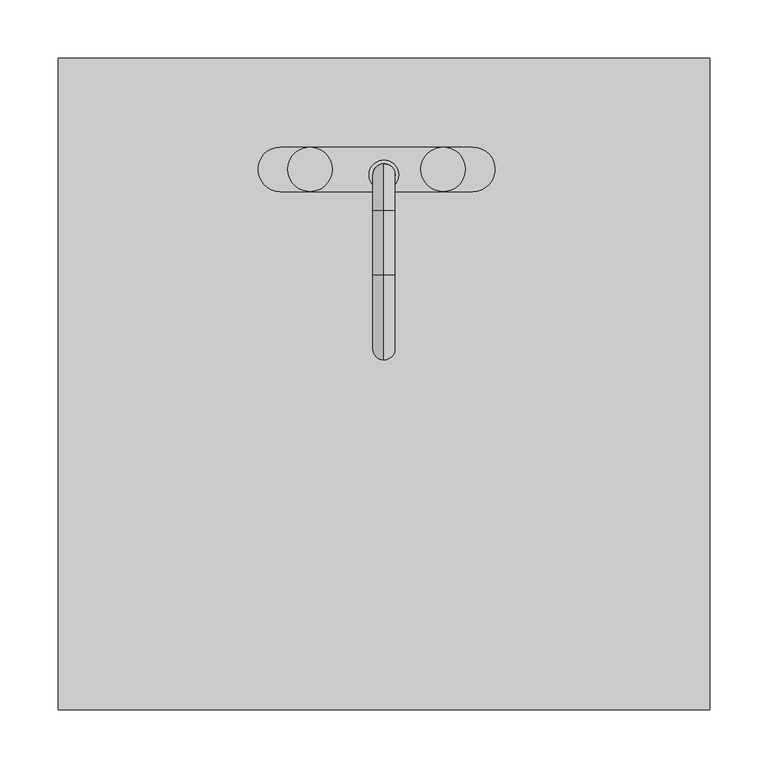
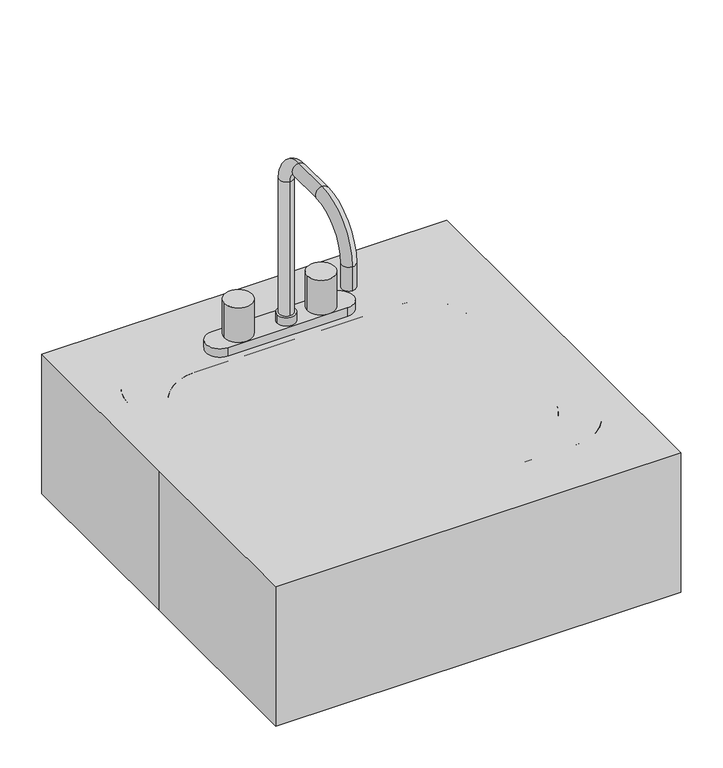
"""IFC4 building model written with IfcOpenShell, lengths in millimetres: proxy geometry, CS090 - Sink, SS, Single Compartment, 7.5x19x16 ID : CS090 - Sink, SS, Single Compartment, 7.5x19x16 ID."""

import ifcopenshell
import ifcopenshell.guid

model = None  # the IFC model being written
_history = None  # IfcOwnerHistory: only IFC2X3 demands one
_inside = {}  # id of a spatial element -> (the spatial element, [elements in it])
_under = {}  # id of a project, library or spatial element -> (it, [spatial elements below it])
_declared = {}  # id of a project -> (the project, [libraries it declares])
_typed = {}  # id of a type object -> (the type object, [elements of that type])
_made_of = {}  # id of a material, layer set ... -> (it, [elements and type objects made of it])


def new_model(schema):
    """Start an empty IFC model of exactly this schema.

    Asked for "IFC4X3", IfcOpenShell would pick the latest addendum, in which some entities
    have other attributes; the version numbers below select the first issue.
    IFC2X3 requires an IfcOwnerHistory on every rooted entity: one is made here for all.
    """
    global model, _history
    if schema == "IFC4X3":
        model = ifcopenshell.file(schema_version=(4, 3, 0, 0))
    else:
        model = ifcopenshell.file(schema=schema)
    _inside.clear()
    _under.clear()
    _declared.clear()
    _typed.clear()
    _made_of.clear()
    _history = None
    if model.schema == "IFC2X3":
        org = make("IfcOrganization", Name="unknown")
        user = make(
            "IfcPersonAndOrganization",
            ThePerson=make("IfcPerson", FamilyName="unknown"),
            TheOrganization=org,
        )
        app = make(
            "IfcApplication",
            ApplicationDeveloper=org,
            Version="unknown",
            ApplicationFullName="unknown",
            ApplicationIdentifier="unknown",
        )
        _history = make(
            "IfcOwnerHistory",
            OwningUser=user,
            OwningApplication=app,
            ChangeAction="ADDED",
            CreationDate=0,
        )
    return model


def make(cls, **values):
    """One entity of the class cls with the attributes given. An attribute that is None is left unset."""
    return model.create_entity(
        cls, **{name: value for name, value in values.items() if value is not None}
    )


def rooted(cls, **values):
    """An entity with a GlobalId (a new one), such as an element, a storey or a relation."""
    return make(cls, GlobalId=ifcopenshell.guid.new(), OwnerHistory=_history, **values)


def si_unit(unit_type, name, prefix=None):
    """IfcSIUnit, for example si_unit("LENGTHUNIT", "METRE", prefix="MILLI")."""
    return make("IfcSIUnit", UnitType=unit_type, Prefix=prefix, Name=name)


def assignment(units):
    """IfcUnitAssignment: the units of a project."""
    return None if units is None else make("IfcUnitAssignment", Units=units)


def point(xyz):
    """IfcCartesianPoint."""
    return None if xyz is None else make("IfcCartesianPoint", Coordinates=xyz)


def direction(xyz):
    """IfcDirection."""
    return None if xyz is None else make("IfcDirection", DirectionRatios=xyz)


def frame(location, z_axis=None, x_axis=None):
    """IfcAxis2Placement3D, a coordinate frame: its origin and axes. An axis left out is left unset."""
    return make(
        "IfcAxis2Placement3D",
        Location=point(location),
        Axis=direction(z_axis),
        RefDirection=direction(x_axis),
    )


def frame_2d(location, x_axis=None):
    """IfcAxis2Placement2D, a coordinate frame in the plane: its origin and x axis."""
    return make(
        "IfcAxis2Placement2D", Location=point(location), RefDirection=direction(x_axis)
    )


def origin():
    """The frame at (0, 0, 0) with its axes left unset."""
    return frame((0.0, 0.0, 0.0))


def origin_with_axes():
    """The frame at (0, 0, 0) with the z axis (0, 0, 1) and the x axis (1, 0, 0) written out."""
    return frame((0.0, 0.0, 0.0), z_axis=(0.0, 0.0, 1.0), x_axis=(1.0, 0.0, 0.0))


def origin_2d():
    """The frame at (0, 0) in the plane with its x axis left unset."""
    return frame_2d((0.0, 0.0))


def place(relative_to, where):
    """IfcLocalPlacement: puts the frame where relative to a parent placement (None: the world)."""
    return make(
        "IfcLocalPlacement", PlacementRelTo=relative_to, RelativePlacement=where
    )


def context(
    kind, dimensions, precision=None, world=None, true_north=None, identifier=None
):
    """IfcGeometricRepresentationContext, for example the 3D "Model" context."""
    return make(
        "IfcGeometricRepresentationContext",
        ContextIdentifier=identifier,
        ContextType=kind,
        CoordinateSpaceDimension=dimensions,
        Precision=precision,
        WorldCoordinateSystem=world,
        TrueNorth=true_north,
    )


def project(units=None, contexts=None):
    """IfcProject with its units and contexts."""
    return rooted(
        "IfcProject",
        Name="project",
        RepresentationContexts=contexts,
        UnitsInContext=assignment(units),
    )


def spatial(cls, under=None, at=None, **own):
    """A site, building, storey or space (cls), placed at a placement, below another one or the project."""
    s = rooted(cls, ObjectPlacement=at, **own)
    if under is not None:
        _under.setdefault(under.id(), (under, []))[1].append(s)
    return s


def polyline(points):
    """IfcPolyline through the points."""
    return make("IfcPolyline", Points=[point(p) for p in points])


def circle_curve(where, radius):
    """IfcCircle in the frame where."""
    return make("IfcCircle", Position=where, Radius=radius)


def ellipse_curve(where, semi_axis1, semi_axis2):
    """IfcEllipse in the frame where."""
    return make(
        "IfcEllipse", Position=where, SemiAxis1=semi_axis1, SemiAxis2=semi_axis2
    )


def trimmed(basis, trim1, trim2, sense, master):
    """IfcTrimmedCurve: the piece of a basis curve between two trims."""
    return make(
        "IfcTrimmedCurve",
        BasisCurve=basis,
        Trim1=trim1,
        Trim2=trim2,
        SenseAgreement=sense,
        MasterRepresentation=master,
    )


def segment(curve, same_sense, transition):
    """IfcCompositeCurveSegment."""
    return make(
        "IfcCompositeCurveSegment",
        Transition=transition,
        SameSense=same_sense,
        ParentCurve=curve,
    )


def composite_curve(segments, self_intersect=None):
    """IfcCompositeCurve: segments joined end to end."""
    return make("IfcCompositeCurve", Segments=segments, SelfIntersect=self_intersect)


def outline(outer, holes=None, kind="AREA"):
    """IfcArbitraryClosedProfileDef: a profile drawn as a closed curve; with holes, ...WithVoids."""
    if holes is None:
        return make("IfcArbitraryClosedProfileDef", ProfileType=kind, OuterCurve=outer)
    return make(
        "IfcArbitraryProfileDefWithVoids",
        ProfileType=kind,
        OuterCurve=outer,
        InnerCurves=holes,
    )


def extrude(swept, where, along, depth):
    """IfcExtrudedAreaSolid: the profile swept, set in the frame where, extruded along a direction by depth."""
    return make(
        "IfcExtrudedAreaSolid",
        SweptArea=swept,
        Position=where,
        ExtrudedDirection=direction(along),
        Depth=depth,
    )


def shape(context_of_items, identifier, shape_type, items):
    """IfcShapeRepresentation: the items that make up one representation, for example the "Body"."""
    return make(
        "IfcShapeRepresentation",
        ContextOfItems=context_of_items,
        RepresentationIdentifier=identifier,
        RepresentationType=shape_type,
        Items=items,
    )


def source(mapping_origin, context_of_items, identifier, shape_type, items):
    """IfcRepresentationMap: a shape defined once, which mapped items show again and again."""
    return make(
        "IfcRepresentationMap",
        MappingOrigin=mapping_origin,
        MappedRepresentation=shape(context_of_items, identifier, shape_type, items),
    )


def transform(
    local_origin,
    x_axis=None,
    y_axis=None,
    z_axis=None,
    scale=None,
    scale2=None,
    scale3=None,
    uniform=True,
):
    """IfcCartesianTransformationOperator3D, or its non-uniform kind. x_axis, y_axis, z_axis: its Axis1, 2, 3."""
    if uniform:
        return make(
            "IfcCartesianTransformationOperator3D",
            Axis1=direction(x_axis),
            Axis2=direction(y_axis),
            LocalOrigin=point(local_origin),
            Scale=scale,
            Axis3=direction(z_axis),
        )
    return make(
        "IfcCartesianTransformationOperator3DnonUniform",
        Axis1=direction(x_axis),
        Axis2=direction(y_axis),
        LocalOrigin=point(local_origin),
        Scale=scale,
        Axis3=direction(z_axis),
        Scale2=scale2,
        Scale3=scale3,
    )


def mapped(mapping_source, mapping_target):
    """IfcMappedItem: shows the shape of a source again, moved by a transform."""
    return make(
        "IfcMappedItem", MappingSource=mapping_source, MappingTarget=mapping_target
    )


def made_of(thing, what):
    """Note that an element or type object is made of a material, layer set ...; save() writes the relation."""
    if what is not None:
        _made_of.setdefault(what.id(), (what, []))[1].append(thing)
    return thing


def element(
    cls,
    number,
    at=None,
    inside=None,
    cuts=None,
    type_object=None,
    material=None,
    context=None,
    identifier="Body",
    shape_type=None,
    held_by="IfcProductDefinitionShape",
    body=None,
    shapes=None,
    **own,
):
    """One element of the class cls, such as IfcWall. Its Tag is "e" and its number.

    at: its placement. inside: the storey or other place that contains it. cuts: it is an
    opening in that element (IfcRelVoidsElement). A single representation is given by context,
    identifier, shape_type and body (its items); several are given by shapes. held_by: the class
    of the entity that holds the representations. save() writes the other relations.
    """
    e = rooted(cls, Tag="e%d" % number, ObjectPlacement=at, **own)
    if body is not None:
        shapes = [shape(context, identifier, shape_type, body)]
    if shapes is not None:
        e.Representation = make(held_by, Representations=shapes)
    if inside is not None:
        _inside.setdefault(inside.id(), (inside, []))[1].append(e)
    if cuts is not None:
        rooted(
            "IfcRelVoidsElement", RelatingBuildingElement=cuts, RelatedOpeningElement=e
        )
    if type_object is not None:
        _typed.setdefault(type_object.id(), (type_object, []))[1].append(e)
    return made_of(e, material)


def aggregate(whole, parts):
    """IfcRelAggregates: a whole, such as a stair, and the parts it consists of."""
    return rooted("IfcRelAggregates", RelatingObject=whole, RelatedObjects=parts)


def save(model, path):
    """Write the relations noted so far, then the file.

    IfcRelAggregates (storeys below a building ...), IfcRelContainedInSpatialStructure (elements
    in a storey), IfcRelDefinesByType, IfcRelAssociatesMaterial and IfcRelDeclares: one each for
    every whole, place, type object, material and project.
    """
    for whole, parts in _under.values():
        aggregate(whole, parts)
    for where, things in _inside.values():
        rooted(
            "IfcRelContainedInSpatialStructure",
            RelatedElements=things,
            RelatingStructure=where,
        )
    for kind, things in _typed.values():
        rooted("IfcRelDefinesByType", RelatedObjects=things, RelatingType=kind)
    for what, things in _made_of.values():
        rooted("IfcRelAssociatesMaterial", RelatedObjects=things, RelatingMaterial=what)
    for by, libraries in _declared.values():
        rooted("IfcRelDeclares", RelatingContext=by, RelatedDefinitions=libraries)
    model.write(path)


def plane_surface(at):
    """IfcPlane: the flat surface through the origin of the frame at, square to its z axis."""
    return make("IfcPlane", Position=at)


def cylinder_surface(at, radius):
    """IfcCylindricalSurface: all points at the distance radius from the z axis of the frame at."""
    return make("IfcCylindricalSurface", Position=at, Radius=radius)


def revolved_surface(curve, axis_point, axis_direction):
    """IfcSurfaceOfRevolution: the curve turned about the line through axis_point along axis_direction."""
    return make(
        "IfcSurfaceOfRevolution",
        SweptCurve=make("IfcArbitraryOpenProfileDef", ProfileType="CURVE", Curve=curve),
        AxisPosition=make("IfcAxis1Placement", Location=point(axis_point), Axis=direction(axis_direction)),
    )


def advanced_brep(points, edges, surfaces, faces):
    """IfcAdvancedBrep: a solid bounded by faces that lie on surfaces and meet in shared edges.

    An edge is (start, end): straight between two places in points (the first is 0);
    or (start, end, curve); or (start, end, curve, False) where it runs against its curve.
    A face is (place in surfaces, loops), or (place, loops, False) where it looks against
    its surface's normal. A loop lists edges by number (the first is 1), with a minus sign
    where the edge is run from its end to its start. The first loop is the outer one.
    """
    corners = [point(p) for p in points]
    vertices = [make("IfcVertexPoint", VertexGeometry=c) for c in corners]
    made = []
    for start, end, *more in edges:
        made.append(
            make(
                "IfcEdgeCurve",
                EdgeStart=vertices[start],
                EdgeEnd=vertices[end],
                EdgeGeometry=more[0] if more else make("IfcPolyline", Points=[corners[start], corners[end]]),
                SameSense=more[1] if len(more) > 1 else True,
            )
        )
    hull = []
    for where, loops, *sense in faces:
        bounds = []
        for j, loop in enumerate(loops):
            ring = [make("IfcOrientedEdge", EdgeElement=made[abs(k) - 1], Orientation=k > 0) for k in loop]
            bounds.append(
                make(
                    "IfcFaceOuterBound" if j == 0 else "IfcFaceBound",
                    Bound=make("IfcEdgeLoop", EdgeList=ring),
                    Orientation=True,
                )
            )
        hull.append(make("IfcAdvancedFace", Bounds=bounds, FaceSurface=surfaces[where], SameSense=sense[0] if sense else True))
    return make("IfcAdvancedBrep", Outer=make("IfcClosedShell", CfsFaces=hull))


def specialty_equipment_25ddf7c5(model_context):
    return source(origin(), model_context, "Body", "SolidModel", [
        extrude(outline(composite_curve([segment(trimmed(circle_curve(frame_2d((139.6999999, 92.075)), 25.4), [point((139.6999999, 117.475))], [point((165.0999999, 92.075))], False, "CARTESIAN"), True, "CONTINUOUS"), segment(polyline([(165.0999999, 92.075), (165.0999999, -101.6)]), True, "CONTINUOUS"), segment(trimmed(circle_curve(frame_2d((139.6999999, -101.6)), 25.4), [point((165.0999999, -101.6))], [point((139.6999999, -127.0))], False, "CARTESIAN"), True, "CONTINUOUS"), segment(polyline([(139.6999999, -127.0), (-139.7000001, -127.0)]), True, "CONTINUOUS"), segment(trimmed(circle_curve(frame_2d((-139.7000001, -101.6)), 25.4), [point((-139.7000001, -127.0))], [point((-165.1000001, -101.6))], False, "CARTESIAN"), True, "CONTINUOUS"), segment(polyline([(-165.1000001, -101.6), (-165.1000001, 92.075)]), True, "CONTINUOUS"), segment(trimmed(circle_curve(frame_2d((-139.7000001, 92.075)), 25.4), [point((-165.1000001, 92.075))], [point((-139.7000001, 117.475))], False, "CARTESIAN"), True, "CONTINUOUS"), segment(polyline([(-139.7000001, 117.475), (139.6999999, 117.475)]), True, "CONTINUOUS")], self_intersect=False), holes=[composite_curve([segment(trimmed(circle_curve(origin_2d(), 12.7), [point((-12.7, 0.0))], [point((12.7, 0.0))], True, "CARTESIAN"), True, "CONTINUOUS"), segment(trimmed(circle_curve(origin_2d(), 12.7), [point((12.7, 0.0))], [point((-12.7, 0.0))], True, "CARTESIAN"), True, "CONTINUOUS")], self_intersect=False)]), origin_with_axes(), (0.0, 0.0, 1.0), 9.525),
        extrude(outline(polyline([(-279.4, 279.4), (279.4, 279.4), (279.4, -279.4), (-279.4, -279.4), (-279.4, 0.0), (-279.4, 279.4)])), origin_with_axes(), (0.0, 0.0, 1.0), 203.2),
        extrude(outline(composite_curve([segment(trimmed(circle_curve(frame_2d((76.1999999, 184.15)), 19.05), [point((76.1999999, 203.2))], [point((76.1999999, 165.1))], False, "CARTESIAN"), True, "CONTINUOUS"), segment(polyline([(76.1999999, 165.1), (-88.9000001, 165.1)]), True, "CONTINUOUS"), segment(trimmed(circle_curve(frame_2d((-88.9000001, 184.15)), 19.05), [point((-88.9000001, 165.1))], [point((-88.9000001, 203.2))], False, "CARTESIAN"), True, "CONTINUOUS"), segment(polyline([(-88.9000001, 203.2), (76.1999999, 203.2)]), True, "CONTINUOUS")], self_intersect=False), holes=[composite_curve([segment(trimmed(circle_curve(frame_2d((-1e-07, 179.3875)), 9.525), [point((-9.5250001, 179.3875))], [point((9.5249999, 179.3875))], True, "CARTESIAN"), True, "CONTINUOUS"), segment(trimmed(circle_curve(frame_2d((-1e-07, 179.3875)), 9.525), [point((9.5249999, 179.3875))], [point((-9.5250001, 179.3875))], True, "CARTESIAN"), True, "CONTINUOUS")], self_intersect=False)]), frame((0.0, 0.0, 203.2), z_axis=(0.0, 0.0, 1.0), x_axis=(1.0, 0.0, 0.0)), (0.0, 0.0, 1.0), 12.7),
        extrude(outline(composite_curve([segment(trimmed(circle_curve(frame_2d((-1e-07, 179.3875)), 12.7), [point((-12.7000001, 179.3875))], [point((12.6999999, 179.3875))], False, "CARTESIAN"), True, "CONTINUOUS"), segment(trimmed(circle_curve(frame_2d((-1e-07, 179.3875)), 12.7), [point((12.6999999, 179.3875))], [point((-12.7000001, 179.3875))], False, "CARTESIAN"), True, "CONTINUOUS")], self_intersect=False), holes=[composite_curve([segment(trimmed(circle_curve(frame_2d((-1e-07, 179.3875)), 9.525), [point((-9.5250001, 179.3875))], [point((9.5249999, 179.3875))], True, "CARTESIAN"), True, "CONTINUOUS"), segment(trimmed(circle_curve(frame_2d((-1e-07, 179.3875)), 9.525), [point((9.5249999, 179.3875))], [point((-9.5250001, 179.3875))], True, "CARTESIAN"), True, "CONTINUOUS")], self_intersect=False)]), frame((0.0, 0.0, 215.9), z_axis=(0.0, 0.0, 1.0), x_axis=(1.0, 0.0, 0.0)), (0.0, 0.0, 1.0), 12.7),
        advanced_brep(
        [(-1e-07, 188.9125, 203.2), (-1e-07, 169.8625, 203.2), (-1e-07, 188.9125, 423.8625), (-1e-07, 169.8625, 423.8625), (-1e-07, 149.225, 444.5), (-1e-07, 149.225, 463.55), (-1e-07, 93.6625, 463.55), (-1e-07, 93.6625, 444.5), (-1e-07, 39.6875, 390.525), (-1e-07, 20.6375, 390.525), (-1e-07, 20.6375, 355.6), (-1e-07, 39.6875, 355.6)],
        [
            (0, 1, circle_curve(frame((-1e-07, 179.3875, 203.2), z_axis=(0.0, 0.0, -1.0), x_axis=(0.0, -1.0, 0.0)), 9.525)),
            (1, 0, circle_curve(frame((-1e-07, 179.3875, 203.2), z_axis=(0.0, 0.0, -1.0), x_axis=(0.0, -1.0, 0.0)), 9.525)),
            (0, 2),
            (2, 3, circle_curve(frame((-1e-07, 179.3875, 423.8625), z_axis=(0.0, 0.0, -1.0), x_axis=(0.0, -1.0, 0.0)), 9.525)),
            (3, 1),
            (3, 2, circle_curve(frame((-1e-07, 179.3875, 423.8625), z_axis=(0.0, 0.0, -1.0), x_axis=(0.0, -1.0, 0.0)), 9.525)),
            (4, 3, circle_curve(frame((-1e-07, 149.225, 423.8625), z_axis=(-1.0, 0.0, 0.0), x_axis=(0.0, 1.0, 0.0)), 20.6375)),
            (2, 5, circle_curve(frame((-1e-07, 149.225, 423.8625), z_axis=(1.0, 0.0, 0.0), x_axis=(0.0, 1.0, 0.0)), 39.6875)),
            (5, 4, circle_curve(frame((-1e-07, 149.225, 454.025), z_axis=(0.0, 1.0, 0.0), x_axis=(0.0, 0.0, -1.0)), 9.525)),
            (4, 5, circle_curve(frame((-1e-07, 149.225, 454.025), z_axis=(0.0, 1.0, 0.0), x_axis=(0.0, 0.0, -1.0)), 9.525)),
            (5, 6),
            (6, 7, circle_curve(frame((-1e-07, 93.6625, 454.025), z_axis=(0.0, 1.0, 0.0), x_axis=(0.0, 0.0, -1.0)), 9.525)),
            (7, 4),
            (7, 6, circle_curve(frame((-1e-07, 93.6625, 454.025), z_axis=(0.0, 1.0, 0.0), x_axis=(0.0, 0.0, -1.0)), 9.525)),
            (8, 7, circle_curve(frame((-1e-07, 93.6625, 390.525), z_axis=(-1.0, 0.0, 0.0), x_axis=(0.0, 0.0, 1.0)), 53.975)),
            (6, 9, circle_curve(frame((-1e-07, 93.6625, 390.525), z_axis=(1.0, 0.0, 0.0), x_axis=(0.0, 0.0, 1.0)), 73.025)),
            (9, 8, circle_curve(frame((-1e-07, 30.1625, 390.525), z_axis=(0.0, 0.0, 1.0), x_axis=(0.0, 1.0, 0.0)), 9.525)),
            (8, 9, circle_curve(frame((-1e-07, 30.1625, 390.525), z_axis=(0.0, 0.0, 1.0), x_axis=(0.0, 1.0, 0.0)), 9.525)),
            (10, 11, circle_curve(frame((-1e-07, 30.1625, 355.6), z_axis=(0.0, 0.0, -1.0), x_axis=(0.0, 1.0, 0.0)), 9.525)),
            (11, 10, circle_curve(frame((-1e-07, 30.1625, 355.6), z_axis=(0.0, 0.0, -1.0), x_axis=(0.0, 1.0, 0.0)), 9.525)),
            (9, 10),
            (11, 8),
        ],
        [
            plane_surface(frame((-1e-07, 169.8625, 203.2), z_axis=(0.0, 0.0, -1.0), x_axis=(1.0, 0.0, 0.0))),
            cylinder_surface(frame((-1e-07, 179.3875, 203.2), z_axis=(0.0, 0.0, -1.0), x_axis=(0.0, -1.0, 0.0)), 9.525),
            revolved_surface(trimmed(ellipse_curve(frame((-1e-07, 179.3875, 423.8625), z_axis=(0.0, 0.0, -1.0), x_axis=(0.0, -1.0, 0.0)), 9.525, 9.525), [point((-1e-07, 188.9125, 423.8625))], [point((-1e-07, 169.8625, 423.8625))], True, "CARTESIAN"), (-1e-07, 149.225, 423.8625), (1.0, 0.0, 0.0)),
            revolved_surface(trimmed(ellipse_curve(frame((-1e-07, 179.3875, 423.8625), z_axis=(0.0, 0.0, -1.0), x_axis=(0.0, -1.0, 0.0)), 9.525, 9.525), [point((-1e-07, 169.8625, 423.8625))], [point((-1e-07, 188.9125, 423.8625))], True, "CARTESIAN"), (-1e-07, 149.225, 423.8625), (1.0, 0.0, 0.0)),
            cylinder_surface(frame((-1e-07, 149.225, 454.025), z_axis=(0.0, 1.0, 0.0), x_axis=(0.0, 0.0, -1.0)), 9.525),
            revolved_surface(trimmed(ellipse_curve(frame((-1e-07, 93.6625, 454.025), z_axis=(0.0, 1.0, 0.0), x_axis=(0.0, 0.0, -1.0)), 9.525, 9.525), [point((-1e-07, 93.6625, 463.55))], [point((-1e-07, 93.6625, 444.5))], True, "CARTESIAN"), (-1e-07, 93.6625, 390.525), (1.0, 0.0, 0.0)),
            revolved_surface(trimmed(ellipse_curve(frame((-1e-07, 93.6625, 454.025), z_axis=(0.0, 1.0, 0.0), x_axis=(0.0, 0.0, -1.0)), 9.525, 9.525), [point((-1e-07, 93.6625, 444.5))], [point((-1e-07, 93.6625, 463.55))], True, "CARTESIAN"), (-1e-07, 93.6625, 390.525), (1.0, 0.0, 0.0)),
            plane_surface(frame((-1e-07, 20.6375, 355.6), z_axis=(0.0, 0.0, -1.0), x_axis=(-1.0, 0.0, 0.0))),
            cylinder_surface(frame((-1e-07, 30.1625, 390.525), z_axis=(0.0, 0.0, 1.0), x_axis=(0.0, 1.0, 0.0)), 9.525),
        ],
        [
            (0, [[1, 2]]),
            (1, [[-1, 3, 4, 5]]),
            (1, [[-2, -5, 6, -3]]),
            (2, [[7, -4, 8, 9]]),
            (3, [[-8, -6, -7, 10]]),
            (4, [[-9, 11, 12, 13]]),
            (4, [[-10, -13, 14, -11]]),
            (5, [[15, -12, 16, 17]]),
            (6, [[-16, -14, -15, 18]]),
            (7, [[19, 20]]),
            (8, [[-17, 21, -20, 22]]),
            (8, [[-18, -22, -19, -21]]),
        ],
    ),
        extrude(outline(composite_curve([segment(trimmed(circle_curve(frame_2d((-63.5000001, 184.15)), 19.05), [point((-82.5500001, 184.15))], [point((-44.4500001, 184.15))], False, "CARTESIAN"), True, "CONTINUOUS"), segment(trimmed(circle_curve(frame_2d((-63.5000001, 184.15)), 19.05), [point((-44.4500001, 184.15))], [point((-82.5500001, 184.15))], False, "CARTESIAN"), True, "CONTINUOUS")], self_intersect=False)), frame((0.0, 0.0, 215.9), z_axis=(0.0, 0.0, 1.0), x_axis=(1.0, 0.0, 0.0)), (0.0, 0.0, 1.0), 50.8),
        extrude(outline(composite_curve([segment(trimmed(circle_curve(frame_2d((50.7999999, 184.15)), 19.05), [point((31.7499999, 184.15))], [point((69.8499999, 184.15))], False, "CARTESIAN"), True, "CONTINUOUS"), segment(trimmed(circle_curve(frame_2d((50.7999999, 184.15)), 19.05), [point((69.8499999, 184.15))], [point((31.7499999, 184.15))], False, "CARTESIAN"), True, "CONTINUOUS")], self_intersect=False)), frame((0.0, 0.0, 215.9), z_axis=(0.0, 0.0, 1.0), x_axis=(1.0, 0.0, 0.0)), (0.0, 0.0, 1.0), 50.8),
        advanced_brep(
        [(-139.7000001, 161.925, 0.0), (-139.7000001, 161.925, 190.5), (139.6999999, 161.925, 190.5), (139.6999999, 161.925, 0.0), (-139.7000001, 117.475, 0.0), (139.6999999, 117.475, 0.0), (-139.7000001, 117.475, 9.525), (139.6999999, 117.475, 9.525), (-139.7000001, 120.0634182, 9.525), (139.6999999, 120.0634182, 9.525), (-139.7000001, 139.0409272, 26.9146831), (139.6999999, 139.0409272, 26.9146831), (-139.7000001, 155.575, 190.5), (139.6999999, 155.575, 190.5), (209.5499999, 92.075, 0.0), (209.5499999, 92.075, 190.5), (165.0999999, 92.075, 0.0), (165.0999999, 92.075, 9.525), (167.6884181, 92.075, 9.525), (186.6659271, 92.075, 26.9146831), (203.1999999, 92.075, 190.5), (209.5499999, -101.6, 190.5), (209.5499999, -101.6, 0.0), (165.0999999, -101.6, 0.0), (165.0999999, -101.6, 9.525), (167.6884181, -101.6, 9.525), (186.6659271, -101.6, 26.9146831), (203.1999999, -101.6, 190.5), (139.6999999, -171.45, 0.0), (139.6999999, -171.45, 190.5), (139.6999999, -127.0, 0.0), (139.6999999, -127.0, 9.525), (139.6999999, -129.5884182, 9.525), (139.6999999, -148.5659272, 26.9146831), (139.6999999, -165.1, 190.5), (-139.7000001, -171.45, 190.5), (-139.7000001, -171.45, 0.0), (-139.7000001, -127.0, 0.0), (-139.7000001, -127.0, 9.525), (-139.7000001, -129.5884182, 9.525), (-139.7000001, -148.5659272, 26.9146831), (-139.7000001, -165.1, 190.5), (-209.5500001, -101.6, 0.0), (-209.5500001, -101.6, 190.5), (-165.1000001, -101.6, 0.0), (-165.1000001, -101.6, 9.525), (-167.6884183, -101.6, 9.525), (-186.6659273, -101.6, 26.9146831), (-203.2000001, -101.6, 190.5), (-209.5500001, 92.075, 190.5), (-209.5500001, 92.075, 0.0), (-165.1000001, 92.075, 0.0), (-165.1000001, 92.075, 9.525), (-167.6884183, 92.075, 9.525), (-186.6659273, 92.075, 26.9146831), (-203.2000001, 92.075, 190.5)],
        [
            (0, 1),
            (1, 2),
            (2, 3),
            (3, 0),
            (4, 0),
            (3, 5),
            (5, 4),
            (6, 4),
            (5, 7),
            (7, 6),
            (8, 6),
            (7, 9),
            (9, 8),
            (10, 8, circle_curve(frame((-139.7000001, 120.0634182, 28.575), z_axis=(-1.0, 0.0, 0.0), x_axis=(0.0, 1.0, 0.0)), 19.05)),
            (9, 11, circle_curve(frame((139.6999999, 120.0634182, 28.575), z_axis=(1.0, 0.0, 0.0), x_axis=(0.0, 1.0, 0.0)), 19.05)),
            (11, 10),
            (12, 10),
            (11, 13),
            (13, 12),
            (1, 12),
            (13, 2),
            (14, 3, circle_curve(frame((139.6999999, 92.075, 0.0), z_axis=(0.0, 0.0, 1.0), x_axis=(0.0, 1.0, 0.0)), 69.85)),
            (2, 15, circle_curve(frame((139.6999999, 92.075, 190.5), z_axis=(0.0, 0.0, -1.0), x_axis=(0.0, 1.0, 0.0)), 69.85)),
            (15, 14),
            (16, 5, circle_curve(frame((139.6999999, 92.075, 0.0), z_axis=(0.0, 0.0, 1.0), x_axis=(0.0, 1.0, 0.0)), 25.4)),
            (14, 16),
            (17, 7, circle_curve(frame((139.6999999, 92.075, 9.525), z_axis=(0.0, 0.0, 1.0), x_axis=(0.0, 1.0, 0.0)), 25.4)),
            (16, 17),
            (18, 9, circle_curve(frame((139.6999999, 92.075, 9.525), z_axis=(0.0, 0.0, 1.0), x_axis=(0.0, 1.0, 0.0)), 27.9884182)),
            (17, 18),
            (19, 11, circle_curve(frame((139.6999999, 92.075, 26.9146831), z_axis=(0.0, 0.0, 1.0), x_axis=(0.0, 1.0, 0.0)), 46.9659272)),
            (18, 19, circle_curve(frame((167.6884181, 92.075, 28.575), z_axis=(0.0, -1.0, 0.0), x_axis=(1.0, 0.0, 0.0)), 19.05)),
            (20, 13, circle_curve(frame((139.6999999, 92.075, 190.5), z_axis=(0.0, 0.0, 1.0), x_axis=(0.0, 1.0, 0.0)), 63.5)),
            (19, 20),
            (20, 15),
            (15, 21),
            (21, 22),
            (22, 14),
            (22, 23),
            (23, 16),
            (23, 24),
            (24, 17),
            (24, 25),
            (25, 18),
            (25, 26, circle_curve(frame((167.6884181, -101.6, 28.575), z_axis=(0.0, -1.0, 0.0), x_axis=(1.0, 0.0, 0.0)), 19.05)),
            (26, 19),
            (26, 27),
            (27, 20),
            (27, 21),
            (28, 22, circle_curve(frame((139.6999999, -101.6, 0.0), z_axis=(0.0, 0.0, 1.0), x_axis=(1.0, 0.0, 0.0)), 69.85)),
            (21, 29, circle_curve(frame((139.6999999, -101.6, 190.5), z_axis=(0.0, 0.0, -1.0), x_axis=(1.0, 0.0, 0.0)), 69.85)),
            (29, 28),
            (30, 23, circle_curve(frame((139.6999999, -101.6, 0.0), z_axis=(0.0, 0.0, 1.0), x_axis=(1.0, 0.0, 0.0)), 25.4)),
            (28, 30),
            (31, 24, circle_curve(frame((139.6999999, -101.6, 9.525), z_axis=(0.0, 0.0, 1.0), x_axis=(1.0, 0.0, 0.0)), 25.4)),
            (30, 31),
            (32, 25, circle_curve(frame((139.6999999, -101.6, 9.525), z_axis=(0.0, 0.0, 1.0), x_axis=(1.0, 0.0, 0.0)), 27.9884182)),
            (31, 32),
            (33, 26, circle_curve(frame((139.6999999, -101.6, 26.9146831), z_axis=(0.0, 0.0, 1.0), x_axis=(1.0, 0.0, 0.0)), 46.9659272)),
            (32, 33, circle_curve(frame((139.6999999, -129.5884182, 28.575), z_axis=(-1.0, 0.0, 0.0), x_axis=(0.0, -1.0, 0.0)), 19.05)),
            (34, 27, circle_curve(frame((139.6999999, -101.6, 190.5), z_axis=(0.0, 0.0, 1.0), x_axis=(1.0, 0.0, 0.0)), 63.5)),
            (33, 34),
            (34, 29),
            (29, 35),
            (35, 36),
            (36, 28),
            (36, 37),
            (37, 30),
            (37, 38),
            (38, 31),
            (38, 39),
            (39, 32),
            (39, 40, circle_curve(frame((-139.7000001, -129.5884182, 28.575), z_axis=(-1.0, 0.0, 0.0), x_axis=(0.0, -1.0, 0.0)), 19.05)),
            (40, 33),
            (40, 41),
            (41, 34),
            (41, 35),
            (42, 36, circle_curve(frame((-139.7000001, -101.6, 0.0), z_axis=(0.0, 0.0, 1.0), x_axis=(0.0, -1.0, 0.0)), 69.85)),
            (35, 43, circle_curve(frame((-139.7000001, -101.6, 190.5), z_axis=(0.0, 0.0, -1.0), x_axis=(0.0, -1.0, 0.0)), 69.85)),
            (43, 42),
            (44, 37, circle_curve(frame((-139.7000001, -101.6, 0.0), z_axis=(0.0, 0.0, 1.0), x_axis=(0.0, -1.0, 0.0)), 25.4)),
            (42, 44),
            (45, 38, circle_curve(frame((-139.7000001, -101.6, 9.525), z_axis=(0.0, 0.0, 1.0), x_axis=(0.0, -1.0, 0.0)), 25.4)),
            (44, 45),
            (46, 39, circle_curve(frame((-139.7000001, -101.6, 9.525), z_axis=(0.0, 0.0, 1.0), x_axis=(0.0, -1.0, 0.0)), 27.9884182)),
            (45, 46),
            (47, 40, circle_curve(frame((-139.7000001, -101.6, 26.9146831), z_axis=(0.0, 0.0, 1.0), x_axis=(0.0, -1.0, 0.0)), 46.9659272)),
            (46, 47, circle_curve(frame((-167.6884183, -101.6, 28.575), z_axis=(0.0, 1.0, 0.0), x_axis=(-1.0, 0.0, 0.0)), 19.05)),
            (48, 41, circle_curve(frame((-139.7000001, -101.6, 190.5), z_axis=(0.0, 0.0, 1.0), x_axis=(0.0, -1.0, 0.0)), 63.5)),
            (47, 48),
            (48, 43),
            (43, 49),
            (49, 50),
            (50, 42),
            (50, 51),
            (51, 44),
            (51, 52),
            (52, 45),
            (52, 53),
            (53, 46),
            (53, 54, circle_curve(frame((-167.6884183, 92.075, 28.575), z_axis=(0.0, 1.0, 0.0), x_axis=(-1.0, 0.0, 0.0)), 19.05)),
            (54, 47),
            (54, 55),
            (55, 48),
            (55, 49),
            (0, 50, circle_curve(frame((-139.7000001, 92.075, 0.0), z_axis=(0.0, 0.0, 1.0), x_axis=(-1.0, 0.0, 0.0)), 69.85)),
            (49, 1, circle_curve(frame((-139.7000001, 92.075, 190.5), z_axis=(0.0, 0.0, -1.0), x_axis=(-1.0, 0.0, 0.0)), 69.85)),
            (4, 51, circle_curve(frame((-139.7000001, 92.075, 0.0), z_axis=(0.0, 0.0, 1.0), x_axis=(-1.0, 0.0, 0.0)), 25.4)),
            (6, 52, circle_curve(frame((-139.7000001, 92.075, 9.525), z_axis=(0.0, 0.0, 1.0), x_axis=(-1.0, 0.0, 0.0)), 25.4)),
            (8, 53, circle_curve(frame((-139.7000001, 92.075, 9.525), z_axis=(0.0, 0.0, 1.0), x_axis=(-1.0, 0.0, 0.0)), 27.9884182)),
            (10, 54, circle_curve(frame((-139.7000001, 92.075, 26.9146831), z_axis=(0.0, 0.0, 1.0), x_axis=(-1.0, 0.0, 0.0)), 46.9659272)),
            (12, 55, circle_curve(frame((-139.7000001, 92.075, 190.5), z_axis=(0.0, 0.0, 1.0), x_axis=(-1.0, 0.0, 0.0)), 63.5)),
        ],
        [
            plane_surface(frame((-139.7000001, 161.925, 190.5), z_axis=(0.0, 1.0, 0.0), x_axis=(1.0, 0.0, 0.0))),
            plane_surface(frame((-139.7000001, 161.925, 0.0), z_axis=(0.0, 0.0, -1.0), x_axis=(1.0, 0.0, 0.0))),
            plane_surface(frame((-139.7000001, 117.475, 0.0), z_axis=(0.0, -1.0, 0.0), x_axis=(1.0, 0.0, 0.0))),
            plane_surface(frame((-139.7000001, 117.475, 9.525), z_axis=(0.0, 0.0, 1.0), x_axis=(1.0, 0.0, 0.0))),
            revolved_surface(polyline([(139.69999989999997, 139.1134182, 28.575), (-139.7000001, 139.1134182, 28.575)]), (-139.7000001, 120.0634182, 28.575), (1.0, 0.0, 0.0)),
            plane_surface(frame((-139.7000001, 139.0409272, 26.9146831), z_axis=(0.0, -0.9949309211512617, 0.10056073854692034), x_axis=(1.0, 0.0, 0.0))),
            plane_surface(frame((-139.7000001, 155.575, 190.5), z_axis=(0.0, 0.0, 1.0), x_axis=(1.0, 0.0, 0.0))),
            cylinder_surface(frame((139.6999999, 92.075, -647.7), z_axis=(0.0, 0.0, -1.0), x_axis=(0.0, 1.0, 0.0)), 69.85),
            plane_surface(frame((139.6999999, 92.075, 0.0), z_axis=(0.0, 0.0, -1.0), x_axis=(0.0, 1.0, 0.0))),
            revolved_surface(polyline([(139.6999999, 117.475, 0.0), (139.6999999, 117.475, 9.524999999999977)]), (139.6999999, 92.075, -647.7), (0.0, 0.0, -1.0)),
            plane_surface(frame((139.6999999, 92.075, 9.525), z_axis=(0.0, 0.0, 1.0), x_axis=(0.0, 1.0, 0.0))),
            revolved_surface(trimmed(ellipse_curve(frame((139.6999999, 120.0634182, 28.575), z_axis=(1.0, 0.0, 0.0), x_axis=(0.0, 1.0, 0.0)), 19.05, 19.05), [point((139.6999999, 120.0634182, 9.525))], [point((139.6999999, 139.0409272, 26.9146831))], True, "CARTESIAN"), (139.6999999, 92.075, -647.7), (0.0, 0.0, -1.0)),
            revolved_surface(polyline([(139.6999999, 139.0409272, 26.9146831), (139.6999999, 155.575, 190.5)]), (139.6999999, 92.075, -647.7), (0.0, 0.0, -1.0)),
            plane_surface(frame((139.6999999, 92.075, 190.5), z_axis=(0.0, 0.0, 1.0), x_axis=(0.0, 1.0, 0.0))),
            plane_surface(frame((209.5499999, 92.075, 190.5), z_axis=(1.0, 0.0, 0.0), x_axis=(0.0, -1.0, 0.0))),
            plane_surface(frame((209.5499999, 92.075, 0.0), z_axis=(0.0, 0.0, -1.0), x_axis=(0.0, -1.0, 0.0))),
            plane_surface(frame((165.0999999, 92.075, 0.0), z_axis=(-1.0, 0.0, 0.0), x_axis=(0.0, -1.0, 0.0))),
            plane_surface(frame((165.0999999, 92.075, 9.525), z_axis=(0.0, 0.0, 1.0), x_axis=(0.0, -1.0, 0.0))),
            revolved_surface(polyline([(186.73841810000002, -101.60000000000001, 28.575), (186.73841810000002, 92.075, 28.575)]), (167.6884181, 92.075, 28.575), (0.0, -1.0, 0.0)),
            plane_surface(frame((186.6659271, 92.075, 26.9146831), z_axis=(-0.9949309211512617, 0.0, 0.10056073854692034), x_axis=(0.0, -1.0, 0.0))),
            plane_surface(frame((203.1999999, 92.075, 190.5), z_axis=(0.0, 0.0, 1.0), x_axis=(0.0, -1.0, 0.0))),
            cylinder_surface(frame((139.6999999, -101.6, -647.7), z_axis=(0.0, 0.0, -1.0), x_axis=(1.0, 0.0, 0.0)), 69.85),
            plane_surface(frame((139.6999999, -101.6, 0.0), z_axis=(0.0, 0.0, -1.0), x_axis=(1.0, 0.0, 0.0))),
            revolved_surface(polyline([(165.0999999, -101.6, 0.0), (165.0999999, -101.6, 9.524999999999977)]), (139.6999999, -101.6, -647.7), (0.0, 0.0, -1.0)),
            plane_surface(frame((139.6999999, -101.6, 9.525), z_axis=(0.0, 0.0, 1.0), x_axis=(1.0, 0.0, 0.0))),
            revolved_surface(trimmed(ellipse_curve(frame((167.6884181, -101.6, 28.575), z_axis=(0.0, -1.0, 0.0), x_axis=(1.0, 0.0, 0.0)), 19.05, 19.05), [point((167.6884181, -101.6, 9.525))], [point((186.6659271, -101.6, 26.9146831))], True, "CARTESIAN"), (139.6999999, -101.6, -647.7), (0.0, 0.0, -1.0)),
            revolved_surface(polyline([(186.6659271, -101.6, 26.9146831), (203.1999999, -101.6, 190.5)]), (139.6999999, -101.6, -647.7), (0.0, 0.0, -1.0)),
            plane_surface(frame((139.6999999, -101.6, 190.5), z_axis=(0.0, 0.0, 1.0), x_axis=(1.0, 0.0, 0.0))),
            plane_surface(frame((139.6999999, -171.45, 190.5), z_axis=(0.0, -1.0, 0.0), x_axis=(-1.0, 0.0, 0.0))),
            plane_surface(frame((139.6999999, -171.45, 0.0), z_axis=(0.0, 0.0, -1.0), x_axis=(-1.0, 0.0, 0.0))),
            plane_surface(frame((139.6999999, -127.0, 0.0), z_axis=(0.0, 1.0, 0.0), x_axis=(-1.0, 0.0, 0.0))),
            plane_surface(frame((139.6999999, -127.0, 9.525), z_axis=(0.0, 0.0, 1.0), x_axis=(-1.0, 0.0, 0.0))),
            revolved_surface(polyline([(-139.70000009999998, -148.63841820000002, 28.575), (139.6999999, -148.63841820000002, 28.575)]), (139.6999999, -129.5884182, 28.575), (-1.0, 0.0, 0.0)),
            plane_surface(frame((139.6999999, -148.5659272, 26.9146831), z_axis=(0.0, 0.9949309211512617, 0.10056073854692034), x_axis=(-1.0, 0.0, 0.0))),
            plane_surface(frame((139.6999999, -165.1, 190.5), z_axis=(0.0, 0.0, 1.0), x_axis=(-1.0, 0.0, 0.0))),
            cylinder_surface(frame((-139.7000001, -101.6, -647.7), z_axis=(0.0, 0.0, -1.0), x_axis=(0.0, -1.0, 0.0)), 69.85),
            plane_surface(frame((-139.7000001, -101.6, 0.0), z_axis=(0.0, 0.0, -1.0), x_axis=(0.0, -1.0, 0.0))),
            revolved_surface(polyline([(-139.7000001, -127.0, 0.0), (-139.7000001, -127.0, 9.524999999999977)]), (-139.7000001, -101.6, -647.7), (0.0, 0.0, -1.0)),
            plane_surface(frame((-139.7000001, -101.6, 9.525), z_axis=(0.0, 0.0, 1.0), x_axis=(0.0, -1.0, 0.0))),
            revolved_surface(trimmed(ellipse_curve(frame((-139.7000001, -129.5884182, 28.575), z_axis=(-1.0, 0.0, 0.0), x_axis=(0.0, -1.0, 0.0)), 19.05, 19.05), [point((-139.7000001, -129.5884182, 9.525))], [point((-139.7000001, -148.5659272, 26.9146831))], True, "CARTESIAN"), (-139.7000001, -101.6, -647.7), (0.0, 0.0, -1.0)),
            revolved_surface(polyline([(-139.7000001, -148.5659272, 26.9146831), (-139.7000001, -165.1, 190.5)]), (-139.7000001, -101.6, -647.7), (0.0, 0.0, -1.0)),
            plane_surface(frame((-139.7000001, -101.6, 190.5), z_axis=(0.0, 0.0, 1.0), x_axis=(0.0, -1.0, 0.0))),
            plane_surface(frame((-209.5500001, -101.6, 190.5), z_axis=(-1.0, 0.0, 0.0), x_axis=(0.0, 1.0, 0.0))),
            plane_surface(frame((-209.5500001, -101.6, 0.0), z_axis=(0.0, 0.0, -1.0), x_axis=(0.0, 1.0, 0.0))),
            plane_surface(frame((-165.1000001, -101.6, 0.0), z_axis=(1.0, 0.0, 0.0), x_axis=(0.0, 1.0, 0.0))),
            plane_surface(frame((-165.1000001, -101.6, 9.525), z_axis=(0.0, 0.0, 1.0), x_axis=(0.0, 1.0, 0.0))),
            revolved_surface(polyline([(-186.7384183, 92.07500000000002, 28.575), (-186.7384183, -101.6, 28.575)]), (-167.6884183, -101.6, 28.575), (0.0, 1.0, 0.0)),
            plane_surface(frame((-186.6659273, -101.6, 26.9146831), z_axis=(0.9949309211512617, 0.0, 0.10056073854692034), x_axis=(0.0, 1.0, 0.0))),
            plane_surface(frame((-203.2000001, -101.6, 190.5), z_axis=(0.0, 0.0, 1.0), x_axis=(0.0, 1.0, 0.0))),
            cylinder_surface(frame((-139.7000001, 92.075, -647.7), z_axis=(0.0, 0.0, -1.0), x_axis=(-1.0, 0.0, 0.0)), 69.85),
            plane_surface(frame((-139.7000001, 92.075, 0.0), z_axis=(0.0, 0.0, -1.0), x_axis=(-1.0, 0.0, 0.0))),
            revolved_surface(polyline([(-165.10000010000002, 92.075, 0.0), (-165.10000010000002, 92.075, 9.524999999999977)]), (-139.7000001, 92.075, -647.7), (0.0, 0.0, -1.0)),
            plane_surface(frame((-139.7000001, 92.075, 9.525), z_axis=(0.0, 0.0, 1.0), x_axis=(-1.0, 0.0, 0.0))),
            revolved_surface(trimmed(ellipse_curve(frame((-167.6884183, 92.075, 28.575), z_axis=(0.0, 1.0, 0.0), x_axis=(-1.0, 0.0, 0.0)), 19.05, 19.05), [point((-167.6884183, 92.075, 9.525))], [point((-186.6659273, 92.075, 26.9146831))], True, "CARTESIAN"), (-139.7000001, 92.075, -647.7), (0.0, 0.0, -1.0)),
            revolved_surface(polyline([(-186.6659273, 92.075, 26.9146831), (-203.2000001, 92.075, 190.5)]), (-139.7000001, 92.075, -647.7), (0.0, 0.0, -1.0)),
            plane_surface(frame((-139.7000001, 92.075, 190.5), z_axis=(0.0, 0.0, 1.0), x_axis=(-1.0, 0.0, 0.0))),
        ],
        [
            (0, [[1, 2, 3, 4]]),
            (1, [[5, -4, 6, 7]]),
            (2, [[8, -7, 9, 10]]),
            (3, [[11, -10, 12, 13]]),
            (4, [[14, -13, 15, 16]]),
            (5, [[17, -16, 18, 19]]),
            (6, [[20, -19, 21, -2]]),
            (7, [[22, -3, 23, 24]]),
            (8, [[25, -6, -22, 26]]),
            (9, [[27, -9, -25, 28]]),
            (10, [[29, -12, -27, 30]]),
            (11, [[31, -15, -29, 32]]),
            (12, [[33, -18, -31, 34]]),
            (13, [[-23, -21, -33, 35]]),
            (14, [[-24, 36, 37, 38]]),
            (15, [[-26, -38, 39, 40]]),
            (16, [[-28, -40, 41, 42]]),
            (17, [[-30, -42, 43, 44]]),
            (18, [[-32, -44, 45, 46]]),
            (19, [[-34, -46, 47, 48]]),
            (20, [[-35, -48, 49, -36]]),
            (21, [[50, -37, 51, 52]]),
            (22, [[53, -39, -50, 54]]),
            (23, [[55, -41, -53, 56]]),
            (24, [[57, -43, -55, 58]]),
            (25, [[59, -45, -57, 60]]),
            (26, [[61, -47, -59, 62]]),
            (27, [[-51, -49, -61, 63]]),
            (28, [[-52, 64, 65, 66]]),
            (29, [[-54, -66, 67, 68]]),
            (30, [[-56, -68, 69, 70]]),
            (31, [[-58, -70, 71, 72]]),
            (32, [[-60, -72, 73, 74]]),
            (33, [[-62, -74, 75, 76]]),
            (34, [[-63, -76, 77, -64]]),
            (35, [[78, -65, 79, 80]]),
            (36, [[81, -67, -78, 82]]),
            (37, [[83, -69, -81, 84]]),
            (38, [[85, -71, -83, 86]]),
            (39, [[87, -73, -85, 88]]),
            (40, [[89, -75, -87, 90]]),
            (41, [[-79, -77, -89, 91]]),
            (42, [[-80, 92, 93, 94]]),
            (43, [[-82, -94, 95, 96]]),
            (44, [[-84, -96, 97, 98]]),
            (45, [[-86, -98, 99, 100]]),
            (46, [[-88, -100, 101, 102]]),
            (47, [[-90, -102, 103, 104]]),
            (48, [[-91, -104, 105, -92]]),
            (49, [[106, -93, 107, -1]]),
            (50, [[108, -95, -106, -5]]),
            (51, [[109, -97, -108, -8]]),
            (52, [[110, -99, -109, -11]]),
            (53, [[111, -101, -110, -14]]),
            (54, [[112, -103, -111, -17]]),
            (55, [[-107, -105, -112, -20]]),
        ],
    ),
        extrude(outline(composite_curve([segment(trimmed(circle_curve(frame_2d((-177.8, -139.7)), 63.5), [point((-177.8, -203.2))], [point((-241.3, -139.7))], False, "CARTESIAN"), True, "CONTINUOUS"), segment(polyline([(-241.3, -139.7), (-241.3, 139.7)]), True, "CONTINUOUS"), segment(trimmed(circle_curve(frame_2d((-177.8, 139.7)), 63.5), [point((-241.3, 139.7))], [point((-177.8, 203.2))], False, "CARTESIAN"), True, "CONTINUOUS"), segment(polyline([(-177.8, 203.2), (177.7999999, 203.2)]), True, "CONTINUOUS"), segment(trimmed(circle_curve(frame_2d((177.7999999, 139.7)), 63.5), [point((177.7999999, 203.2))], [point((241.2999999, 139.7))], False, "CARTESIAN"), True, "CONTINUOUS"), segment(polyline([(241.2999999, 139.7), (241.2999999, -139.7)]), True, "CONTINUOUS"), segment(trimmed(circle_curve(frame_2d((177.7999999, -139.7)), 63.5), [point((241.2999999, -139.7))], [point((177.7999999, -203.2))], False, "CARTESIAN"), True, "CONTINUOUS"), segment(polyline([(177.7999999, -203.2), (-177.8, -203.2)]), True, "CONTINUOUS")], self_intersect=False), holes=[composite_curve([segment(polyline([(139.6999999, 155.575), (-139.7000001, 155.575)]), True, "CONTINUOUS"), segment(trimmed(circle_curve(frame_2d((-139.7000001, 92.075)), 63.5), [point((-139.7000001, 155.575))], [point((-203.2000001, 92.075))], True, "CARTESIAN"), True, "CONTINUOUS"), segment(polyline([(-203.2000001, 92.075), (-203.2000001, -101.6)]), True, "CONTINUOUS"), segment(trimmed(circle_curve(frame_2d((-139.7000001, -101.6)), 63.5), [point((-203.2000001, -101.6))], [point((-139.7000001, -165.1))], True, "CARTESIAN"), True, "CONTINUOUS"), segment(polyline([(-139.7000001, -165.1), (139.6999999, -165.1)]), True, "CONTINUOUS"), segment(trimmed(circle_curve(frame_2d((139.6999999, -101.6)), 63.5), [point((139.6999999, -165.1))], [point((203.1999999, -101.6))], True, "CARTESIAN"), True, "CONTINUOUS"), segment(polyline([(203.1999999, -101.6), (203.1999999, 92.075)]), True, "CONTINUOUS"), segment(trimmed(circle_curve(frame_2d((139.6999999, 92.075)), 63.5), [point((203.1999999, 92.075))], [point((139.6999999, 155.575))], True, "CARTESIAN"), True, "CONTINUOUS")], self_intersect=False)]), frame((0.0, 0.0, 190.5), z_axis=(0.0, 0.0, 1.0), x_axis=(1.0, 0.0, 0.0)), (0.0, 0.0, 1.0), 12.7),
    ])


if __name__ == "__main__":
    model = new_model("IFC4")
    model_context = context("Model", 3, world=origin())
    ifc_project = project(units=[si_unit("LENGTHUNIT", "METRE", prefix="MILLI")], contexts=[model_context])
    site = spatial("IfcSite", under=ifc_project)
    building = spatial("IfcBuilding", under=site)
    placement = place(None, origin())
    specialty_equipment_shape = specialty_equipment_25ddf7c5(model_context)
    element("IfcBuildingElementProxy", 1, Name="CS090 - Sink, SS, Single Compartment, 7.5x19x16 ID : CS090 - Sink, SS, Single Compartment, 7.5x19x16 ID", ObjectType="CS090 - Sink, SS, Single Compartment, 7.5x19x16 ID : CS090 - Sink, SS, Single Compartment, 7.5x19x16 ID", at=placement, inside=building, context=model_context, shape_type="MappedRepresentation", body=[
        mapped(specialty_equipment_shape, transform((0.0, 0.0, 0.0), x_axis=(1.0, 0.0, 0.0), y_axis=(0.0, 1.0, 0.0), z_axis=(0.0, 0.0, 1.0))),
    ])
    save(model, "model.ifc")

# Revit data of these elements
# Type "CS090 - Sink, SS, Single Compartment, 7.5x19x16 ID : CS090 - Sink, SS, Single Compartment, 7.5x19x16 ID"
#   Watts2 = "0"
#   Watts1 = "0"
#   Unit_Issue = "EA"
#   UTIL_6_Misc = "-"
#   UTIL_5_NonMedGas = "-"
#   UTIL_4_MiscGas = "-"
#   UTIL_3_MedGas = "-"
#   UTIL_2_Elec = "-"
#   UTIL_1_WaterDrain = "D"
#   Nomenclature = "Sink, SS, Single Compartment, 7.5x19x16 ID"
#   NSN = "6530"
#   Location [instance default] = ""
#   JSN = "CS090"
#   Fund_Source_VA = "-"
#   Fund_Source_Navy = "-"
#   Fund_Source_Army = "-"
#   Fund_Source_AF = "-"
#   ELEC_Volts2 = "0"
#   ELEC_Volts1 = "0"
#   ELEC_Phase2 = "0"
#   ELEC_Phase1 = "0"
#   ELEC_HertzSwitch = "0"
#   ELEC_HertzDependent = "0"
#   ELEC_Hertz = "0"
#   ELEC_Amps2 = "0"
#   ELEC_Amps1 = "0"
#   DetailDescription = "Single compartment stainless steel sink, drop-in, self-rimming, ledge-type, connected with a drain and provided with a mixing faucet. It shall also be provided with pre-punched fixture holes on 4\" center, integral back ledge to accommodate deck-mounted fixtures, brushed/polished interior and top surfaces, and sound deadened. Recommended for use in suspended or U/C/B sink cabinets having a high plastic laminate or Chemsurf laminate countertop/work surface. Coordinate actual outside sink dimensions with the actual clear dimension of cabinet specified to ensure that they are compatible. For general purpose use throughout the facility."
#   CAT_VA = "A"
#   CAT_Navy = "A"
#   CAT_IHS = "-"
#   CAT_Army = "A"
#   CAT_AF = "A"
#   BTUperhour = "0"
#   Weight_IP = 27
#   DIM_Width_IP = 1' - 10"
#   DIM_Height_IP = 0' - 8"
#   DIM_Depth_IP = 1' - 10"
#   Faucet Material = Metal - Steel, Polished
#   Basin Material = Default
#   Assembly Code = ""
# Element 1 (IfcBuildingElementProxy, "CS090 - Sink, SS, Single Compartment, 7.5x19x16 ID : CS090 - Sink, SS, Single Compartment, 7.5x19x16 ID")
#   Location = "DNPL2"
#   Materials on its faces: "Default", "Metal - Steel, Polished", "EquipSpace"
# Materials
#   "Metal - Steel, Polished": class "Unassigned", colour RGB 57 57 57, transparency 0
#   "Default": class "Miscellaneous", colour RGB 127 127 127, transparency 0
#   "EquipSpace": class "Unassigned", colour RGB 221 217 195, transparency 0.5
